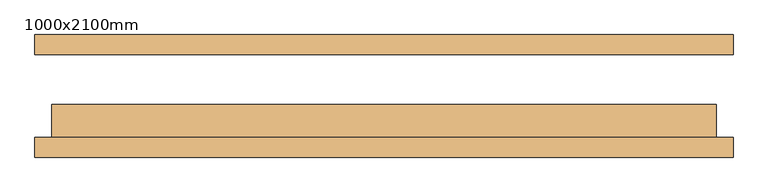
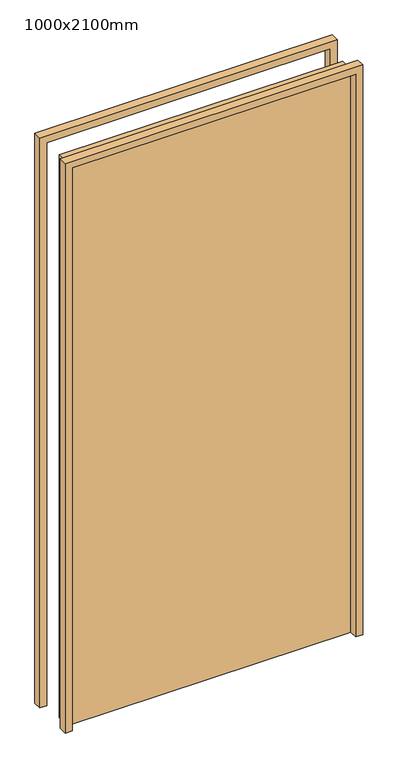
"""IFC4 building model written with IfcOpenShell, lengths in millimetres: door geometry, WWm-SingleSolid-Flush : 1000x2100mm."""

from ifc_helpers import new_model, si_unit, frame, origin, origin_with_axes, place, context, project, spatial, polyline, outline, extrude, source, transform, mapped, element, save


def door_1000x2100mm_40c70491(model_context):
    return source(origin(), model_context, "Body", "SweptSolid", [
        extrude(outline(polyline([(2125.0, -525.0), (0.0, -525.0), (0.0, -500.0), (2100.0, -500.0), (2100.0, 500.0), (0.0, 500.0), (0.0, 525.0), (2125.0, 525.0), (2125.0, -525.0)])), frame((0.0, -92.5, 0.0), z_axis=(0.0, 1.0, 0.0), x_axis=(0.0, 0.0, 1.0)), (0.0, 0.0, 1.0), 30.0),
        extrude(outline(polyline([(2125.0, 525.0), (2125.0, -525.0), (0.0, -525.0), (0.0, -500.0), (2100.0, -500.0), (2100.0, 500.0), (0.0, 500.0), (0.0, 525.0), (2125.0, 525.0)])), frame((0.0, 62.5, 0.0), z_axis=(0.0, 1.0, 0.0), x_axis=(0.0, 0.0, 1.0)), (0.0, 0.0, 1.0), 30.0),
        extrude(outline(polyline([(500.0, -12.5), (500.0, -62.5), (-500.0, -62.5), (-500.0, -12.5), (500.0, -12.5)])), origin_with_axes(), (0.0, 0.0, 1.0), 2100.0),
    ])


if __name__ == "__main__":
    model = new_model("IFC4")
    model_context = context("Model", 3, world=origin())
    ifc_project = project(units=[si_unit("LENGTHUNIT", "METRE", prefix="MILLI")], contexts=[model_context])
    site = spatial("IfcSite", under=ifc_project)
    building = spatial("IfcBuilding", under=site)
    placement = place(None, origin())
    door_1000x2100mm_shape = door_1000x2100mm_40c70491(model_context)
    element("IfcDoor", 1, ObjectType="WWm-SingleSolid-Flush : 1000x2100mm", at=placement, inside=building, context=model_context, shape_type="MappedRepresentation", body=[
        mapped(door_1000x2100mm_shape, transform((0.0, 0.0, 0.0), x_axis=(1.0, 0.0, 0.0), y_axis=(0.0, 1.0, 0.0), z_axis=(0.0, 0.0, 1.0))),
    ])
    save(model, "model.ifc")

# Revit data of these elements
# Type "WWm-SingleSolid-Flush : 1000x2100mm"
#   Type Mark = "EX1-51"
#   Construction Type Id = "MDOOR"
#   Assembly Code = "C1020"
#   Analytic Construction = "Metal"
#   Thickness = 50 mm
#   Thermal Resistance (R) = 0.270117 (m²·K)/W
#   Heat Transfer Coefficient (U) = 3.7021 W/(m²·K)
#   Height = 2100 mm
#   Trim Projection Ext = 30 mm
#   Trim Projection Int = 30 mm
#   Trim Width = 25 mm
#   Width = 1000 mm
#   Not 90 Degree [instance default] = no
#   90 Degree [instance default] = yes
#   Door Material = WW-EC-RGB-White
#   Frame Material = WW-EC-RGB-White
#   Visual Light Transmittance = 0
#   Solar Heat Gain Coefficient = 0
#   Function = (empty or 0)
#   Wall Closure = (empty or 0)
# Element 1 (IfcDoor, "WWm-SingleSolid-Flush : 1000x2100mm")
#   Materials on its faces: "WW-EC-RGB-White"
# Materials
#   "WW-EC-RGB-White": class "Generic", colour RGB 255 255 255, transparency 0, Comments = "If region requests off-white, swith asset color to RGB 231-228-220", Description = "Generic Color", Cost = 0
